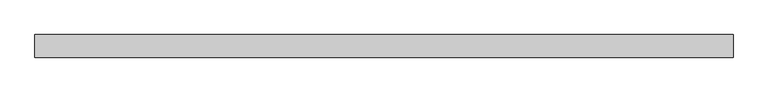
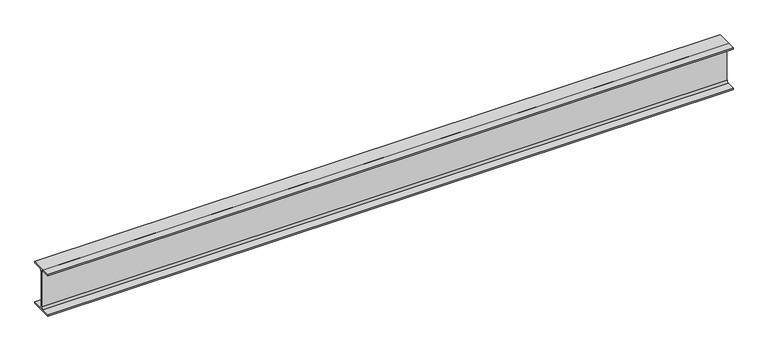
"""IFC4 building model written with IfcOpenShell, lengths in millimetres: beam geometry, 0912_Steel Framing_H-KSD3502 : H_SB_ASB_H-250x125x6x9."""

from ifc_helpers import new_model, si_unit, point, frame, frame_2d, origin, place, context, project, spatial, polyline, circle_curve, trimmed, segment, composite_curve, outline, extrude, source, transform, mapped, element, save


def beam_437020b8(model_context):
    return source(origin(), model_context, "Body", "SweptSolid", [
        extrude(outline(composite_curve([segment(polyline([(62.5, -116.0), (62.5, -125.0), (-62.5, -125.0), (-62.5, -116.0), (-15.0, -116.0)]), True, "CONTINUOUS"), segment(trimmed(circle_curve(frame_2d((-15.0, -104.0)), 12.0), [point((-15.0, -116.0))], [point((-3.0, -104.0))], True, "CARTESIAN"), True, "CONTINUOUS"), segment(polyline([(-3.0, -104.0), (-3.0, 104.0)]), True, "CONTINUOUS"), segment(trimmed(circle_curve(frame_2d((-15.0, 104.0)), 12.0), [point((-3.0, 104.0))], [point((-15.0, 116.0))], True, "CARTESIAN"), True, "CONTINUOUS"), segment(polyline([(-15.0, 116.0), (-62.5, 116.0), (-62.5, 125.0), (62.5, 125.0), (62.5, 116.0), (15.0, 116.0)]), True, "CONTINUOUS"), segment(trimmed(circle_curve(frame_2d((15.0, 104.0)), 12.0), [point((15.0, 116.0))], [point((3.0, 104.0))], True, "CARTESIAN"), True, "CONTINUOUS"), segment(polyline([(3.0, 104.0), (3.0, -104.0)]), True, "CONTINUOUS"), segment(trimmed(circle_curve(frame_2d((15.0, -104.0)), 12.0), [point((3.0, -104.0))], [point((15.0, -116.0))], True, "CARTESIAN"), True, "CONTINUOUS"), segment(polyline([(15.0, -116.0), (62.5, -116.0)]), True, "CONTINUOUS")], self_intersect=False)), frame((-2029.8, 0.0, 0.0), z_axis=(1.0, 0.0, 0.0), x_axis=(0.0, 1.0, 0.0)), (0.0, 0.0, 1.0), 3859.8827532),
    ])


if __name__ == "__main__":
    model = new_model("IFC4")
    model_context = context("Model", 3, world=origin())
    ifc_project = project(units=[si_unit("LENGTHUNIT", "METRE", prefix="MILLI")], contexts=[model_context])
    site = spatial("IfcSite", under=ifc_project)
    building = spatial("IfcBuilding", under=site)
    placement = place(None, origin())
    beam_shape = beam_437020b8(model_context)
    element("IfcBeam", 1, ObjectType="0912_Steel Framing_H-KSD3502 : H_SB_ASB_H-250x125x6x9", at=placement, inside=building, context=model_context, shape_type="MappedRepresentation", body=[
        mapped(beam_shape, transform((0.0, 0.0, 0.0), x_axis=(1.0, 0.0, 0.0), y_axis=(0.0, 1.0, 0.0), z_axis=(0.0, 0.0, 1.0))),
    ])
    save(model, "model.ifc")

# Revit data of these elements
# Type "0912_Steel Framing_H-KSD3502 : H_SB_ASB_H-250x125x6x9"
#   H_WM Code_1 = "S01AA003-00001 | Main Steel Structure Fabrication Work | Shelter/Building | Light Steel - Standard (30KG/M>Weight) | Material: (   )"
#   H_WM Code_2 = "S03AA029-00001 | Main Steel Structure Erection Work | Shelter/Building | Light Steel (30KG/M>Weight) | Material: (   )"
#   H_WM Code_3 = "S01AA010-00001 | Main Steel Structure Fabrication Work | Shelter/Building | Steel Painting/Coating | for Non-Fireproofed Steel Surface, Surface Preparation, Primer, Second & Final Coat | Material: (   )"
#   H_Q'ty Cal Type Tag = "SB-Q2"
#   Width = 12.5 cm
#   Web Thickness = 0.6 cm
#   Web Fillet = 1.2 cm
#   Warping Constant = 42539.8 cm⁶
#   W = 0
#   Torsional Moment of Inertia = 7.8102 cm⁴
#   Section Area = 37.66 cm²
#   Plastic Modulus weak axis = 73.1 cm³
#   Plastic Modulus strong axis = 366.0 cm³
#   Perimeter = 0.97 m²/m
#   Nominal Weight = 29.60 kgf/m
#   Moment of Inertia weak axis = 294.00 cm⁴
#   Moment of Inertia strong axis = 4050.00 cm⁴
#   Height = 25.0 cm
#   Flange Thickness = 0.9 cm
#   Elastic Modulus weak axis = 47.0 cm³
#   Elastic Modulus strong axis = 324.0 cm³
#   Centroid Vertical = 12.5 cm
#   Centroid Horizontal = 6.25 cm
#   Ix = 40500000
#   Length [instance default] = 1.5240 m
#   Zx = 366000
#   b = 0.1250 m
#   h = 0.2500 m
#   r = 0.0120 m
#   s = 0.0060 m
#   t = 0.0090 m
#   A = 0.003766 m²
#   Structural Material [instance default] = Steel, 45-345
#   Assembly Code = ""
# Element 1 (IfcBeam, "0912_Steel Framing_H-KSD3502 : H_SB_ASB_H-250x125x6x9")
#   Structural Material = none
# Materials
#   "Steel, 45-345": class "Metal", colour RGB 189 187 185, transparency 0, Description = "Steel 345 MPa", Cost = 0
